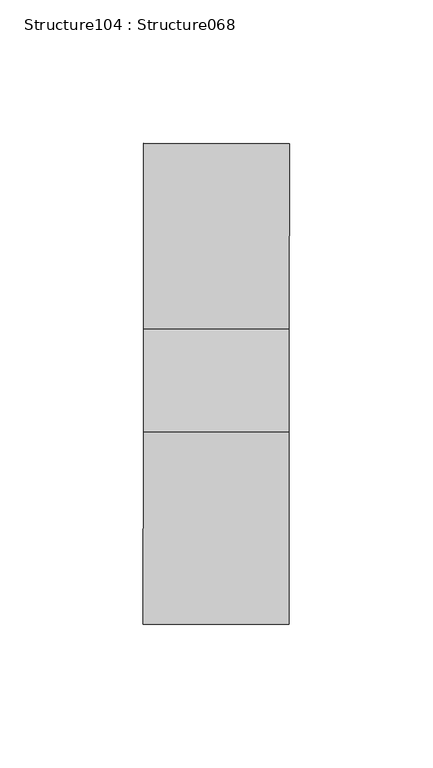
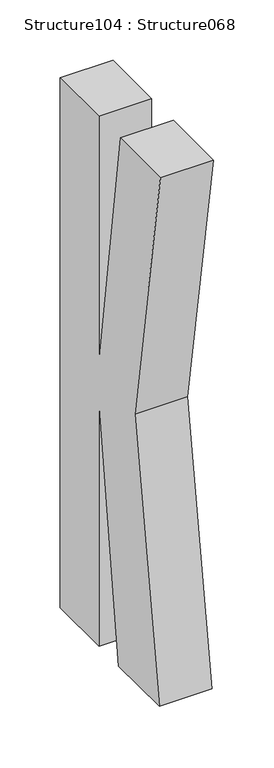
"""IFC4 building model written with IfcOpenShell, lengths in millimetres: proxy geometry, Structure104 : Structure068."""

from ifc_helpers import new_model, si_unit, frame, origin, place, context, project, spatial, polyline, outline, extrude, source, transform, mapped, element, save


def structure104_structure068_b5fe51e2(model_context):
    return source(origin(), model_context, "Body", "SweptSolid", [
        extrude(outline(polyline([(274.9994632, 0.0), (264.9886588, -66.8596998), (13.921021, -62.6677254), (260.0973798, -99.5273491), (250.5395907, -163.3614714), (-281.3127819, -83.7279988), (-271.7549927, -19.8938765), (-24.8238231, -56.8665169), (-266.4085382, 15.8137778), (-256.511172, 81.9158516), (0.0, 0.0), (274.9994632, 0.0)])), frame((-56111.4118908, 291501.3627702, 105.171671), z_axis=(-0.9999998917542984, 0.00046528635450596156, 0.0), x_axis=(-6.889861504106206e-05, -0.14807785983899338, -0.9889757037857322)), (0.0, 0.0, 1.0), 50.8),
    ])


if __name__ == "__main__":
    model = new_model("IFC4")
    model_context = context("Model", 3, world=origin())
    ifc_project = project(units=[si_unit("LENGTHUNIT", "METRE", prefix="MILLI")], contexts=[model_context])
    site = spatial("IfcSite", under=ifc_project)
    building = spatial("IfcBuilding", under=site)
    placement = place(None, origin())
    structure104_structure068_shape = structure104_structure068_b5fe51e2(model_context)
    element("IfcBuildingElementProxy", 1, Name="Structure104 : Structure068", ObjectType="Structure104 : Structure068", at=placement, inside=building, context=model_context, shape_type="MappedRepresentation", body=[
        mapped(structure104_structure068_shape, transform((0.0, 0.0, 0.0), x_axis=(1.0, 0.0, 0.0), y_axis=(0.0, 1.0, 0.0), z_axis=(0.0, 0.0, 1.0))),
    ])
    save(model, "model.ifc")

# Revit data of these elements
# Type "Structure104 : Structure068"
#   NameOverride = "Structure068"
# Element 1 (IfcBuildingElementProxy, "Structure104 : Structure068")
#   Materials on its faces: "BRUSHED ALUMINUM LETTERING"
# Materials
#   "BRUSHED ALUMINUM LETTERING": class "Unassigned", colour RGB 169 181 186, transparency 0, Cost = 0
